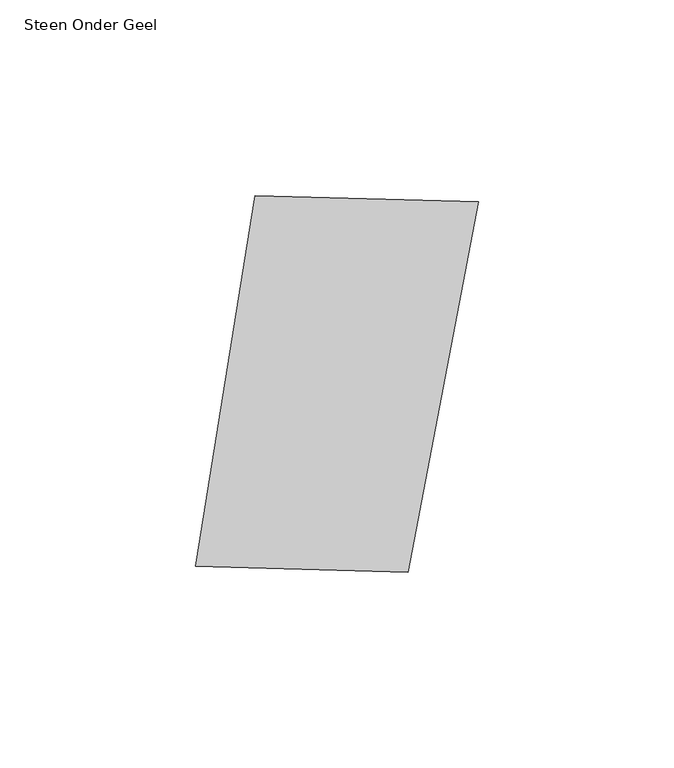
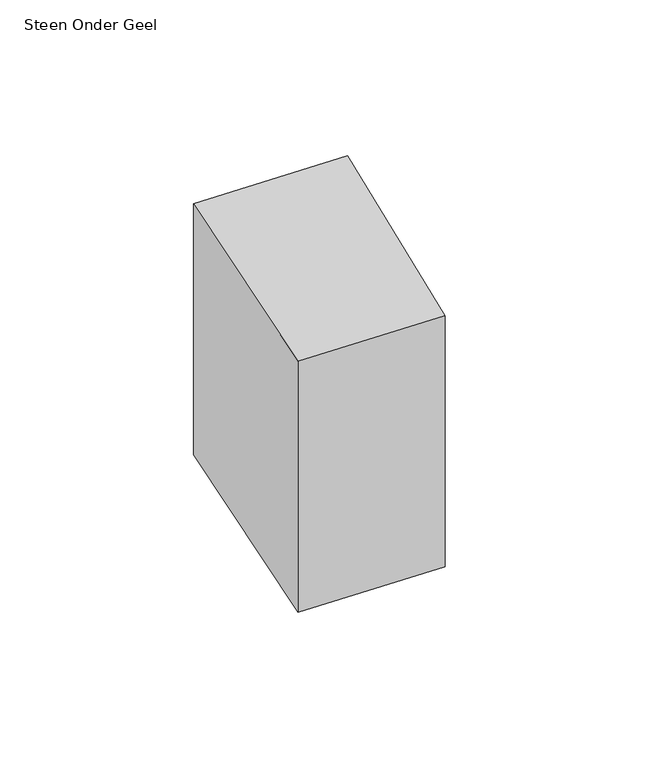
"""IFC4 building model written with IfcOpenShell, lengths in millimetres: proxy geometry, 00_GMA_steen_versie_4 : Steen Onder Geel."""

import ifcopenshell
import ifcopenshell.guid

model = None  # the IFC model being written
_history = None  # IfcOwnerHistory: only IFC2X3 demands one
_inside = {}  # id of a spatial element -> (the spatial element, [elements in it])
_under = {}  # id of a project, library or spatial element -> (it, [spatial elements below it])
_declared = {}  # id of a project -> (the project, [libraries it declares])
_typed = {}  # id of a type object -> (the type object, [elements of that type])
_made_of = {}  # id of a material, layer set ... -> (it, [elements and type objects made of it])


def new_model(schema):
    """Start an empty IFC model of exactly this schema.

    Asked for "IFC4X3", IfcOpenShell would pick the latest addendum, in which some entities
    have other attributes; the version numbers below select the first issue.
    IFC2X3 requires an IfcOwnerHistory on every rooted entity: one is made here for all.
    """
    global model, _history
    if schema == "IFC4X3":
        model = ifcopenshell.file(schema_version=(4, 3, 0, 0))
    else:
        model = ifcopenshell.file(schema=schema)
    _inside.clear()
    _under.clear()
    _declared.clear()
    _typed.clear()
    _made_of.clear()
    _history = None
    if model.schema == "IFC2X3":
        org = make("IfcOrganization", Name="unknown")
        user = make(
            "IfcPersonAndOrganization",
            ThePerson=make("IfcPerson", FamilyName="unknown"),
            TheOrganization=org,
        )
        app = make(
            "IfcApplication",
            ApplicationDeveloper=org,
            Version="unknown",
            ApplicationFullName="unknown",
            ApplicationIdentifier="unknown",
        )
        _history = make(
            "IfcOwnerHistory",
            OwningUser=user,
            OwningApplication=app,
            ChangeAction="ADDED",
            CreationDate=0,
        )
    return model


def make(cls, **values):
    """One entity of the class cls with the attributes given. An attribute that is None is left unset."""
    return model.create_entity(
        cls, **{name: value for name, value in values.items() if value is not None}
    )


def rooted(cls, **values):
    """An entity with a GlobalId (a new one), such as an element, a storey or a relation."""
    return make(cls, GlobalId=ifcopenshell.guid.new(), OwnerHistory=_history, **values)


def si_unit(unit_type, name, prefix=None):
    """IfcSIUnit, for example si_unit("LENGTHUNIT", "METRE", prefix="MILLI")."""
    return make("IfcSIUnit", UnitType=unit_type, Prefix=prefix, Name=name)


def assignment(units):
    """IfcUnitAssignment: the units of a project."""
    return None if units is None else make("IfcUnitAssignment", Units=units)


def point(xyz):
    """IfcCartesianPoint."""
    return None if xyz is None else make("IfcCartesianPoint", Coordinates=xyz)


def direction(xyz):
    """IfcDirection."""
    return None if xyz is None else make("IfcDirection", DirectionRatios=xyz)


def frame(location, z_axis=None, x_axis=None):
    """IfcAxis2Placement3D, a coordinate frame: its origin and axes. An axis left out is left unset."""
    return make(
        "IfcAxis2Placement3D",
        Location=point(location),
        Axis=direction(z_axis),
        RefDirection=direction(x_axis),
    )


def origin():
    """The frame at (0, 0, 0) with its axes left unset."""
    return frame((0.0, 0.0, 0.0))


def origin_with_axes():
    """The frame at (0, 0, 0) with the z axis (0, 0, 1) and the x axis (1, 0, 0) written out."""
    return frame((0.0, 0.0, 0.0), z_axis=(0.0, 0.0, 1.0), x_axis=(1.0, 0.0, 0.0))


def place(relative_to, where):
    """IfcLocalPlacement: puts the frame where relative to a parent placement (None: the world)."""
    return make(
        "IfcLocalPlacement", PlacementRelTo=relative_to, RelativePlacement=where
    )


def context(
    kind, dimensions, precision=None, world=None, true_north=None, identifier=None
):
    """IfcGeometricRepresentationContext, for example the 3D "Model" context."""
    return make(
        "IfcGeometricRepresentationContext",
        ContextIdentifier=identifier,
        ContextType=kind,
        CoordinateSpaceDimension=dimensions,
        Precision=precision,
        WorldCoordinateSystem=world,
        TrueNorth=true_north,
    )


def project(units=None, contexts=None):
    """IfcProject with its units and contexts."""
    return rooted(
        "IfcProject",
        Name="project",
        RepresentationContexts=contexts,
        UnitsInContext=assignment(units),
    )


def spatial(cls, under=None, at=None, **own):
    """A site, building, storey or space (cls), placed at a placement, below another one or the project."""
    s = rooted(cls, ObjectPlacement=at, **own)
    if under is not None:
        _under.setdefault(under.id(), (under, []))[1].append(s)
    return s


def polyline(points):
    """IfcPolyline through the points."""
    return make("IfcPolyline", Points=[point(p) for p in points])


def outline(outer, holes=None, kind="AREA"):
    """IfcArbitraryClosedProfileDef: a profile drawn as a closed curve; with holes, ...WithVoids."""
    if holes is None:
        return make("IfcArbitraryClosedProfileDef", ProfileType=kind, OuterCurve=outer)
    return make(
        "IfcArbitraryProfileDefWithVoids",
        ProfileType=kind,
        OuterCurve=outer,
        InnerCurves=holes,
    )


def extrude(swept, where, along, depth):
    """IfcExtrudedAreaSolid: the profile swept, set in the frame where, extruded along a direction by depth."""
    return make(
        "IfcExtrudedAreaSolid",
        SweptArea=swept,
        Position=where,
        ExtrudedDirection=direction(along),
        Depth=depth,
    )


def shape(context_of_items, identifier, shape_type, items):
    """IfcShapeRepresentation: the items that make up one representation, for example the "Body"."""
    return make(
        "IfcShapeRepresentation",
        ContextOfItems=context_of_items,
        RepresentationIdentifier=identifier,
        RepresentationType=shape_type,
        Items=items,
    )


def source(mapping_origin, context_of_items, identifier, shape_type, items):
    """IfcRepresentationMap: a shape defined once, which mapped items show again and again."""
    return make(
        "IfcRepresentationMap",
        MappingOrigin=mapping_origin,
        MappedRepresentation=shape(context_of_items, identifier, shape_type, items),
    )


def transform(
    local_origin,
    x_axis=None,
    y_axis=None,
    z_axis=None,
    scale=None,
    scale2=None,
    scale3=None,
    uniform=True,
):
    """IfcCartesianTransformationOperator3D, or its non-uniform kind. x_axis, y_axis, z_axis: its Axis1, 2, 3."""
    if uniform:
        return make(
            "IfcCartesianTransformationOperator3D",
            Axis1=direction(x_axis),
            Axis2=direction(y_axis),
            LocalOrigin=point(local_origin),
            Scale=scale,
            Axis3=direction(z_axis),
        )
    return make(
        "IfcCartesianTransformationOperator3DnonUniform",
        Axis1=direction(x_axis),
        Axis2=direction(y_axis),
        LocalOrigin=point(local_origin),
        Scale=scale,
        Axis3=direction(z_axis),
        Scale2=scale2,
        Scale3=scale3,
    )


def mapped(mapping_source, mapping_target):
    """IfcMappedItem: shows the shape of a source again, moved by a transform."""
    return make(
        "IfcMappedItem", MappingSource=mapping_source, MappingTarget=mapping_target
    )


def made_of(thing, what):
    """Note that an element or type object is made of a material, layer set ...; save() writes the relation."""
    if what is not None:
        _made_of.setdefault(what.id(), (what, []))[1].append(thing)
    return thing


def element(
    cls,
    number,
    at=None,
    inside=None,
    cuts=None,
    type_object=None,
    material=None,
    context=None,
    identifier="Body",
    shape_type=None,
    held_by="IfcProductDefinitionShape",
    body=None,
    shapes=None,
    **own,
):
    """One element of the class cls, such as IfcWall. Its Tag is "e" and its number.

    at: its placement. inside: the storey or other place that contains it. cuts: it is an
    opening in that element (IfcRelVoidsElement). A single representation is given by context,
    identifier, shape_type and body (its items); several are given by shapes. held_by: the class
    of the entity that holds the representations. save() writes the other relations.
    """
    e = rooted(cls, Tag="e%d" % number, ObjectPlacement=at, **own)
    if body is not None:
        shapes = [shape(context, identifier, shape_type, body)]
    if shapes is not None:
        e.Representation = make(held_by, Representations=shapes)
    if inside is not None:
        _inside.setdefault(inside.id(), (inside, []))[1].append(e)
    if cuts is not None:
        rooted(
            "IfcRelVoidsElement", RelatingBuildingElement=cuts, RelatedOpeningElement=e
        )
    if type_object is not None:
        _typed.setdefault(type_object.id(), (type_object, []))[1].append(e)
    return made_of(e, material)


def aggregate(whole, parts):
    """IfcRelAggregates: a whole, such as a stair, and the parts it consists of."""
    return rooted("IfcRelAggregates", RelatingObject=whole, RelatedObjects=parts)


def save(model, path):
    """Write the relations noted so far, then the file.

    IfcRelAggregates (storeys below a building ...), IfcRelContainedInSpatialStructure (elements
    in a storey), IfcRelDefinesByType, IfcRelAssociatesMaterial and IfcRelDeclares: one each for
    every whole, place, type object, material and project.
    """
    for whole, parts in _under.values():
        aggregate(whole, parts)
    for where, things in _inside.values():
        rooted(
            "IfcRelContainedInSpatialStructure",
            RelatedElements=things,
            RelatingStructure=where,
        )
    for kind, things in _typed.values():
        rooted("IfcRelDefinesByType", RelatedObjects=things, RelatingType=kind)
    for what, things in _made_of.values():
        rooted("IfcRelAssociatesMaterial", RelatedObjects=things, RelatingMaterial=what)
    for by, libraries in _declared.values():
        rooted("IfcRelDeclares", RelatingContext=by, RelatedDefinitions=libraries)
    model.write(path)


def steen_onder_geel_801346a3(model_context):
    return source(origin(), model_context, "Body", "SweptSolid", [
        extrude(outline(polyline([(109.0791109, 113.5760365), (91.0973663, 18.9875051), (36.8116594, 20.5326468), (52.0125313, 115.1827189), (109.0791109, 113.5760365)])), origin_with_axes(), (0.0, 0.0, 1.0), 100.0),
    ])


if __name__ == "__main__":
    model = new_model("IFC4")
    model_context = context("Model", 3, world=origin())
    ifc_project = project(units=[si_unit("LENGTHUNIT", "METRE", prefix="MILLI")], contexts=[model_context])
    site = spatial("IfcSite", under=ifc_project)
    building = spatial("IfcBuilding", under=site)
    placement = place(None, origin())
    steen_onder_geel_shape = steen_onder_geel_801346a3(model_context)
    element("IfcBuildingElementProxy", 1, Name="00_GMA_steen_versie_4 : Steen Onder Geel", ObjectType="00_GMA_steen_versie_4 : Steen Onder Geel", at=placement, inside=building, context=model_context, shape_type="MappedRepresentation", body=[
        mapped(steen_onder_geel_shape, transform((0.0, 0.0, 0.0), x_axis=(1.0, 0.0, 0.0), y_axis=(0.0, 1.0, 0.0), z_axis=(0.0, 0.0, 1.0))),
    ])
    save(model, "model.ifc")

# Revit data of these elements
# Type "00_GMA_steen_versie_4 : Steen Onder Geel"
#   StootVoegHalfBoven [instance default] = 5 mm
#   StootVoegHalf [instance default] = 5 mm
#   StootVoegBreedteOnder = 10 mm
#   StootVoegBreedteBoven = 10 mm
#   Steendikte = 100 mm
#   LintVoegOnderHalf = 0 mm
#   LintVoegOnder = 0 mm
#   LintVoegBovenHalf = 5 mm
#   LintVoegBoven = 10 mm
#   materiaal = 21_steen_geel
#   MateriaalVoeg = none
#   Default Elevation = 0
# Element 1 (IfcBuildingElementProxy, "00_GMA_steen_versie_4 : Steen Onder Geel")
#   Materials on its faces: "21_steen_geel"
# Materials
#   "21_steen_geel": class "Unassigned", colour RGB 202 202 0, transparency 0, Cost = 0
